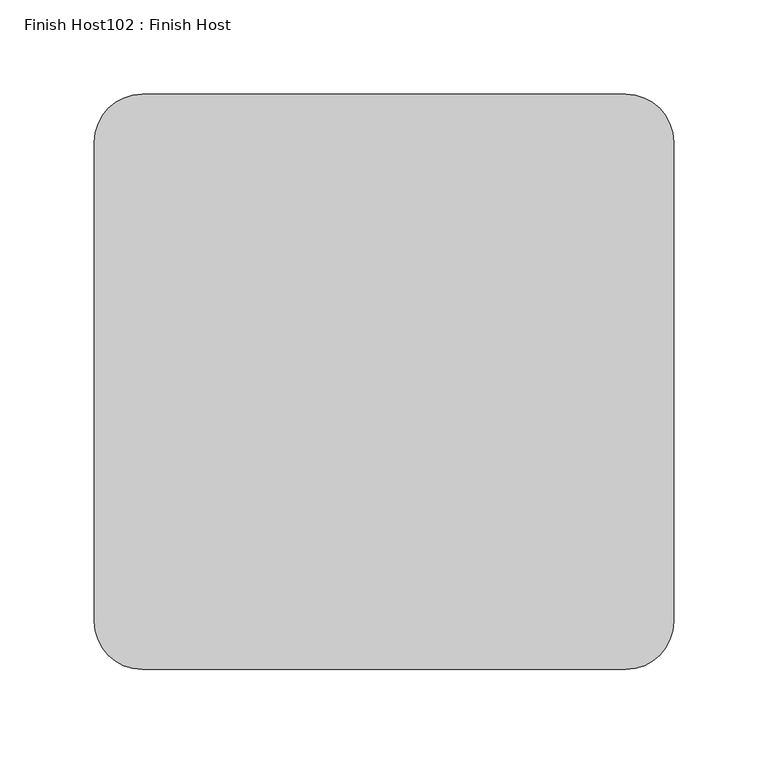
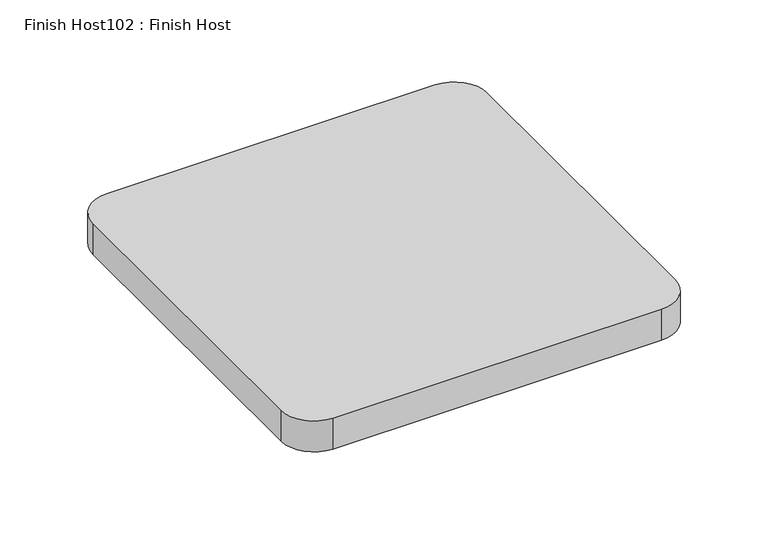
"""IFC4 building model written with IfcOpenShell, lengths in millimetres: proxy geometry, Finish Host102 : Finish Host."""

import ifcopenshell
import ifcopenshell.guid

model = None  # the IFC model being written
_history = None  # IfcOwnerHistory: only IFC2X3 demands one
_inside = {}  # id of a spatial element -> (the spatial element, [elements in it])
_under = {}  # id of a project, library or spatial element -> (it, [spatial elements below it])
_declared = {}  # id of a project -> (the project, [libraries it declares])
_typed = {}  # id of a type object -> (the type object, [elements of that type])
_made_of = {}  # id of a material, layer set ... -> (it, [elements and type objects made of it])


def new_model(schema):
    """Start an empty IFC model of exactly this schema.

    Asked for "IFC4X3", IfcOpenShell would pick the latest addendum, in which some entities
    have other attributes; the version numbers below select the first issue.
    IFC2X3 requires an IfcOwnerHistory on every rooted entity: one is made here for all.
    """
    global model, _history
    if schema == "IFC4X3":
        model = ifcopenshell.file(schema_version=(4, 3, 0, 0))
    else:
        model = ifcopenshell.file(schema=schema)
    _inside.clear()
    _under.clear()
    _declared.clear()
    _typed.clear()
    _made_of.clear()
    _history = None
    if model.schema == "IFC2X3":
        org = make("IfcOrganization", Name="unknown")
        user = make(
            "IfcPersonAndOrganization",
            ThePerson=make("IfcPerson", FamilyName="unknown"),
            TheOrganization=org,
        )
        app = make(
            "IfcApplication",
            ApplicationDeveloper=org,
            Version="unknown",
            ApplicationFullName="unknown",
            ApplicationIdentifier="unknown",
        )
        _history = make(
            "IfcOwnerHistory",
            OwningUser=user,
            OwningApplication=app,
            ChangeAction="ADDED",
            CreationDate=0,
        )
    return model


def make(cls, **values):
    """One entity of the class cls with the attributes given. An attribute that is None is left unset."""
    return model.create_entity(
        cls, **{name: value for name, value in values.items() if value is not None}
    )


def rooted(cls, **values):
    """An entity with a GlobalId (a new one), such as an element, a storey or a relation."""
    return make(cls, GlobalId=ifcopenshell.guid.new(), OwnerHistory=_history, **values)


def si_unit(unit_type, name, prefix=None):
    """IfcSIUnit, for example si_unit("LENGTHUNIT", "METRE", prefix="MILLI")."""
    return make("IfcSIUnit", UnitType=unit_type, Prefix=prefix, Name=name)


def assignment(units):
    """IfcUnitAssignment: the units of a project."""
    return None if units is None else make("IfcUnitAssignment", Units=units)


def point(xyz):
    """IfcCartesianPoint."""
    return None if xyz is None else make("IfcCartesianPoint", Coordinates=xyz)


def direction(xyz):
    """IfcDirection."""
    return None if xyz is None else make("IfcDirection", DirectionRatios=xyz)


def frame(location, z_axis=None, x_axis=None):
    """IfcAxis2Placement3D, a coordinate frame: its origin and axes. An axis left out is left unset."""
    return make(
        "IfcAxis2Placement3D",
        Location=point(location),
        Axis=direction(z_axis),
        RefDirection=direction(x_axis),
    )


def frame_2d(location, x_axis=None):
    """IfcAxis2Placement2D, a coordinate frame in the plane: its origin and x axis."""
    return make(
        "IfcAxis2Placement2D", Location=point(location), RefDirection=direction(x_axis)
    )


def origin():
    """The frame at (0, 0, 0) with its axes left unset."""
    return frame((0.0, 0.0, 0.0))


def origin_with_axes():
    """The frame at (0, 0, 0) with the z axis (0, 0, 1) and the x axis (1, 0, 0) written out."""
    return frame((0.0, 0.0, 0.0), z_axis=(0.0, 0.0, 1.0), x_axis=(1.0, 0.0, 0.0))


def place(relative_to, where):
    """IfcLocalPlacement: puts the frame where relative to a parent placement (None: the world)."""
    return make(
        "IfcLocalPlacement", PlacementRelTo=relative_to, RelativePlacement=where
    )


def context(
    kind, dimensions, precision=None, world=None, true_north=None, identifier=None
):
    """IfcGeometricRepresentationContext, for example the 3D "Model" context."""
    return make(
        "IfcGeometricRepresentationContext",
        ContextIdentifier=identifier,
        ContextType=kind,
        CoordinateSpaceDimension=dimensions,
        Precision=precision,
        WorldCoordinateSystem=world,
        TrueNorth=true_north,
    )


def project(units=None, contexts=None):
    """IfcProject with its units and contexts."""
    return rooted(
        "IfcProject",
        Name="project",
        RepresentationContexts=contexts,
        UnitsInContext=assignment(units),
    )


def spatial(cls, under=None, at=None, **own):
    """A site, building, storey or space (cls), placed at a placement, below another one or the project."""
    s = rooted(cls, ObjectPlacement=at, **own)
    if under is not None:
        _under.setdefault(under.id(), (under, []))[1].append(s)
    return s


def polyline(points):
    """IfcPolyline through the points."""
    return make("IfcPolyline", Points=[point(p) for p in points])


def circle_curve(where, radius):
    """IfcCircle in the frame where."""
    return make("IfcCircle", Position=where, Radius=radius)


def trimmed(basis, trim1, trim2, sense, master):
    """IfcTrimmedCurve: the piece of a basis curve between two trims."""
    return make(
        "IfcTrimmedCurve",
        BasisCurve=basis,
        Trim1=trim1,
        Trim2=trim2,
        SenseAgreement=sense,
        MasterRepresentation=master,
    )


def segment(curve, same_sense, transition):
    """IfcCompositeCurveSegment."""
    return make(
        "IfcCompositeCurveSegment",
        Transition=transition,
        SameSense=same_sense,
        ParentCurve=curve,
    )


def composite_curve(segments, self_intersect=None):
    """IfcCompositeCurve: segments joined end to end."""
    return make("IfcCompositeCurve", Segments=segments, SelfIntersect=self_intersect)


def outline(outer, holes=None, kind="AREA"):
    """IfcArbitraryClosedProfileDef: a profile drawn as a closed curve; with holes, ...WithVoids."""
    if holes is None:
        return make("IfcArbitraryClosedProfileDef", ProfileType=kind, OuterCurve=outer)
    return make(
        "IfcArbitraryProfileDefWithVoids",
        ProfileType=kind,
        OuterCurve=outer,
        InnerCurves=holes,
    )


def extrude(swept, where, along, depth):
    """IfcExtrudedAreaSolid: the profile swept, set in the frame where, extruded along a direction by depth."""
    return make(
        "IfcExtrudedAreaSolid",
        SweptArea=swept,
        Position=where,
        ExtrudedDirection=direction(along),
        Depth=depth,
    )


def shape(context_of_items, identifier, shape_type, items):
    """IfcShapeRepresentation: the items that make up one representation, for example the "Body"."""
    return make(
        "IfcShapeRepresentation",
        ContextOfItems=context_of_items,
        RepresentationIdentifier=identifier,
        RepresentationType=shape_type,
        Items=items,
    )


def source(mapping_origin, context_of_items, identifier, shape_type, items):
    """IfcRepresentationMap: a shape defined once, which mapped items show again and again."""
    return make(
        "IfcRepresentationMap",
        MappingOrigin=mapping_origin,
        MappedRepresentation=shape(context_of_items, identifier, shape_type, items),
    )


def transform(
    local_origin,
    x_axis=None,
    y_axis=None,
    z_axis=None,
    scale=None,
    scale2=None,
    scale3=None,
    uniform=True,
):
    """IfcCartesianTransformationOperator3D, or its non-uniform kind. x_axis, y_axis, z_axis: its Axis1, 2, 3."""
    if uniform:
        return make(
            "IfcCartesianTransformationOperator3D",
            Axis1=direction(x_axis),
            Axis2=direction(y_axis),
            LocalOrigin=point(local_origin),
            Scale=scale,
            Axis3=direction(z_axis),
        )
    return make(
        "IfcCartesianTransformationOperator3DnonUniform",
        Axis1=direction(x_axis),
        Axis2=direction(y_axis),
        LocalOrigin=point(local_origin),
        Scale=scale,
        Axis3=direction(z_axis),
        Scale2=scale2,
        Scale3=scale3,
    )


def mapped(mapping_source, mapping_target):
    """IfcMappedItem: shows the shape of a source again, moved by a transform."""
    return make(
        "IfcMappedItem", MappingSource=mapping_source, MappingTarget=mapping_target
    )


def made_of(thing, what):
    """Note that an element or type object is made of a material, layer set ...; save() writes the relation."""
    if what is not None:
        _made_of.setdefault(what.id(), (what, []))[1].append(thing)
    return thing


def element(
    cls,
    number,
    at=None,
    inside=None,
    cuts=None,
    type_object=None,
    material=None,
    context=None,
    identifier="Body",
    shape_type=None,
    held_by="IfcProductDefinitionShape",
    body=None,
    shapes=None,
    **own,
):
    """One element of the class cls, such as IfcWall. Its Tag is "e" and its number.

    at: its placement. inside: the storey or other place that contains it. cuts: it is an
    opening in that element (IfcRelVoidsElement). A single representation is given by context,
    identifier, shape_type and body (its items); several are given by shapes. held_by: the class
    of the entity that holds the representations. save() writes the other relations.
    """
    e = rooted(cls, Tag="e%d" % number, ObjectPlacement=at, **own)
    if body is not None:
        shapes = [shape(context, identifier, shape_type, body)]
    if shapes is not None:
        e.Representation = make(held_by, Representations=shapes)
    if inside is not None:
        _inside.setdefault(inside.id(), (inside, []))[1].append(e)
    if cuts is not None:
        rooted(
            "IfcRelVoidsElement", RelatingBuildingElement=cuts, RelatedOpeningElement=e
        )
    if type_object is not None:
        _typed.setdefault(type_object.id(), (type_object, []))[1].append(e)
    return made_of(e, material)


def aggregate(whole, parts):
    """IfcRelAggregates: a whole, such as a stair, and the parts it consists of."""
    return rooted("IfcRelAggregates", RelatingObject=whole, RelatedObjects=parts)


def save(model, path):
    """Write the relations noted so far, then the file.

    IfcRelAggregates (storeys below a building ...), IfcRelContainedInSpatialStructure (elements
    in a storey), IfcRelDefinesByType, IfcRelAssociatesMaterial and IfcRelDeclares: one each for
    every whole, place, type object, material and project.
    """
    for whole, parts in _under.values():
        aggregate(whole, parts)
    for where, things in _inside.values():
        rooted(
            "IfcRelContainedInSpatialStructure",
            RelatedElements=things,
            RelatingStructure=where,
        )
    for kind, things in _typed.values():
        rooted("IfcRelDefinesByType", RelatedObjects=things, RelatingType=kind)
    for what, things in _made_of.values():
        rooted("IfcRelAssociatesMaterial", RelatedObjects=things, RelatingMaterial=what)
    for by, libraries in _declared.values():
        rooted("IfcRelDeclares", RelatingContext=by, RelatedDefinitions=libraries)
    model.write(path)


def finish_host102_finish_host_9602d006(model_context):
    return source(origin(), model_context, "Body", "SweptSolid", [
        extrude(outline(composite_curve([segment(polyline([(-799.2083644, 4229.4760864), (-799.2083644, 4483.4760864)]), True, "CONTINUOUS"), segment(trimmed(circle_curve(frame_2d((-773.8083644, 4483.4760864)), 25.4), [point((-799.2083644, 4483.4760864))], [point((-773.8083644, 4508.8760864))], False, "CARTESIAN"), True, "CONTINUOUS"), segment(polyline([(-773.8083644, 4508.8760864), (-517.7842816, 4508.8760864)]), True, "CONTINUOUS"), segment(trimmed(circle_curve(frame_2d((-517.7842816, 4483.4760864)), 25.4), [point((-517.7842816, 4508.8760864))], [point((-492.3842816, 4483.4760864))], False, "CARTESIAN"), True, "CONTINUOUS"), segment(polyline([(-492.3842816, 4483.4760864), (-492.3842816, 4229.4760864)]), True, "CONTINUOUS"), segment(trimmed(circle_curve(frame_2d((-517.7842816, 4229.4760864)), 25.4), [point((-492.3842816, 4229.4760864))], [point((-517.7842816, 4204.0760864))], False, "CARTESIAN"), True, "CONTINUOUS"), segment(polyline([(-517.7842816, 4204.0760864), (-773.8083644, 4204.0760864)]), True, "CONTINUOUS"), segment(trimmed(circle_curve(frame_2d((-773.8083644, 4229.4760864)), 25.4), [point((-773.8083644, 4204.0760864))], [point((-799.2083644, 4229.4760864))], False, "CARTESIAN"), True, "CONTINUOUS")], self_intersect=False)), origin_with_axes(), (0.0, 0.0, 1.0), 25.4),
    ])


if __name__ == "__main__":
    model = new_model("IFC4")
    model_context = context("Model", 3, world=origin())
    ifc_project = project(units=[si_unit("LENGTHUNIT", "METRE", prefix="MILLI")], contexts=[model_context])
    site = spatial("IfcSite", under=ifc_project)
    building = spatial("IfcBuilding", under=site)
    placement = place(None, origin())
    finish_host102_finish_host_shape = finish_host102_finish_host_9602d006(model_context)
    element("IfcBuildingElementProxy", 1, Name="Finish Host102 : Finish Host", ObjectType="Finish Host102 : Finish Host", at=placement, inside=building, context=model_context, shape_type="MappedRepresentation", body=[
        mapped(finish_host102_finish_host_shape, transform((0.0, 0.0, 0.0), x_axis=(1.0, 0.0, 0.0), y_axis=(0.0, 1.0, 0.0), z_axis=(0.0, 0.0, 1.0))),
    ])
    save(model, "model.ifc")

# Revit data of these elements
# Type "Finish Host102 : Finish Host"
#   Panel Material = Fabric - Teknion - G100 - Homage - Respect
# Element 1 (IfcBuildingElementProxy, "Finish Host102 : Finish Host")
#   Materials on its faces: "Fabric - Teknion - G100 - Homage - Respect"
# Materials
#   "Fabric - Teknion - G100 - Homage - Respect": class "Generic", colour RGB 99 95 90, transparency 0, Model = "G100", Manufacturer = "Teknion Studio", URL = "http://www.teknionstudio.com/", Description = "Respect Homage", Cost = 0
